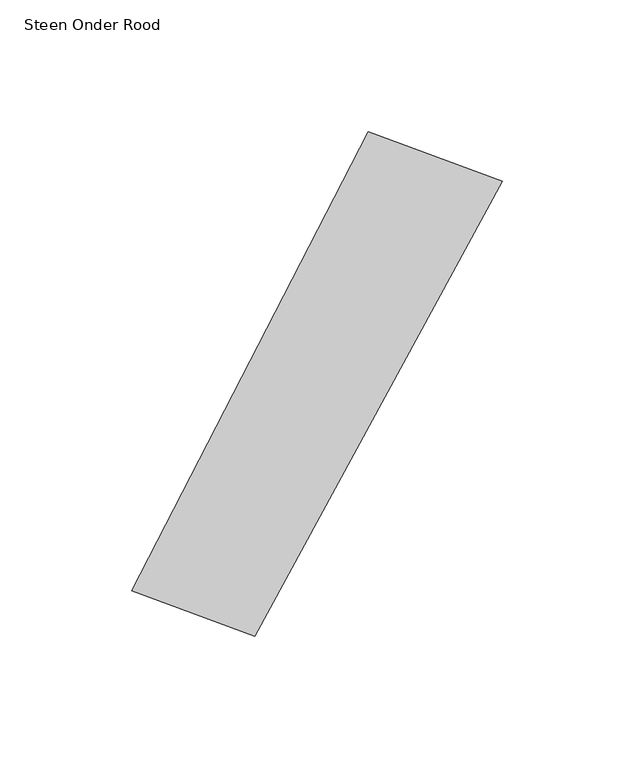
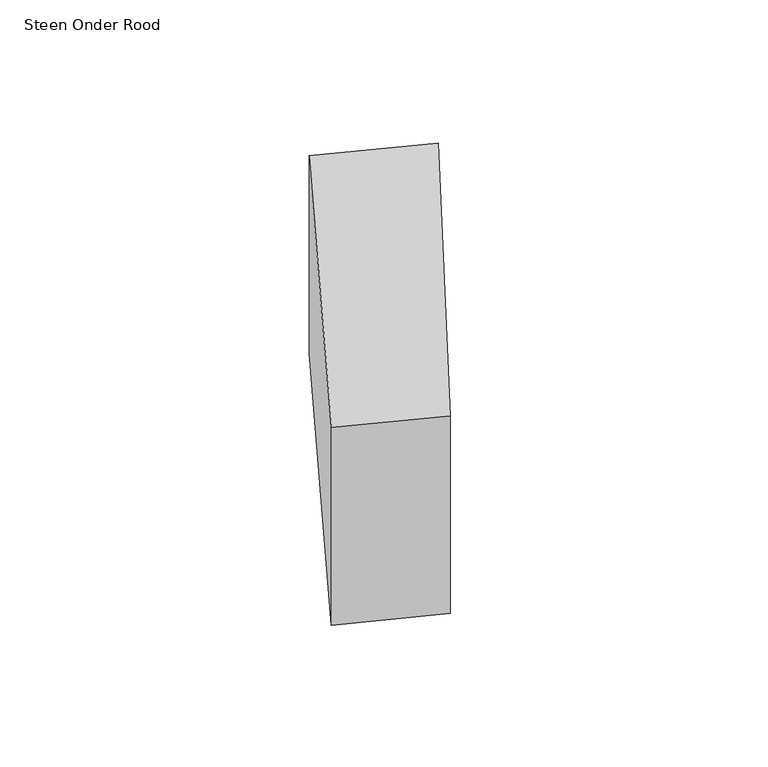
"""IFC4 building model written with IfcOpenShell, lengths in millimetres: proxy geometry, 00_GMA_steen_versie_4 : Steen Onder Rood."""

from ifc_helpers import new_model, si_unit, origin, origin_with_axes, place, context, project, spatial, polyline, outline, extrude, source, transform, mapped, element, save


def steen_onder_rood_62b55ba9(model_context):
    return source(origin(), model_context, "Body", "SweptSolid", [
        extrude(outline(polyline([(146.7402477, 154.7030668), (52.5992174, -18.4322574), (5.7094797, -1.0727499), (95.7797788, 173.5566477), (146.7402477, 154.7030668)])), origin_with_axes(), (0.0, 0.0, 1.0), 100.0),
    ])


if __name__ == "__main__":
    model = new_model("IFC4")
    model_context = context("Model", 3, world=origin())
    ifc_project = project(units=[si_unit("LENGTHUNIT", "METRE", prefix="MILLI")], contexts=[model_context])
    site = spatial("IfcSite", under=ifc_project)
    building = spatial("IfcBuilding", under=site)
    placement = place(None, origin())
    steen_onder_rood_shape = steen_onder_rood_62b55ba9(model_context)
    element("IfcBuildingElementProxy", 1, Name="00_GMA_steen_versie_4 : Steen Onder Rood", ObjectType="00_GMA_steen_versie_4 : Steen Onder Rood", at=placement, inside=building, context=model_context, shape_type="MappedRepresentation", body=[
        mapped(steen_onder_rood_shape, transform((0.0, 0.0, 0.0), x_axis=(1.0, 0.0, 0.0), y_axis=(0.0, 1.0, 0.0), z_axis=(0.0, 0.0, 1.0))),
    ])
    save(model, "model.ifc")

# Revit data of these elements
# Type "00_GMA_steen_versie_4 : Steen Onder Rood"
#   StootVoegHalfBoven [instance default] = 5 mm
#   StootVoegHalf [instance default] = 5 mm
#   StootVoegBreedteOnder = 10 mm
#   StootVoegBreedteBoven = 10 mm
#   Steendikte = 100 mm
#   LintVoegOnderHalf = 0 mm
#   LintVoegOnder = 0 mm
#   LintVoegBovenHalf = 5 mm
#   LintVoegBoven = 10 mm
#   materiaal = 21_steen_rood
#   MateriaalVoeg = none
#   Default Elevation = 0
# Element 1 (IfcBuildingElementProxy, "00_GMA_steen_versie_4 : Steen Onder Rood")
#   Materials on its faces: "21_steen_rood"
# Materials
#   "21_steen_rood": class "Unassigned", colour RGB 213 111 43, transparency 0, Cost = 0
